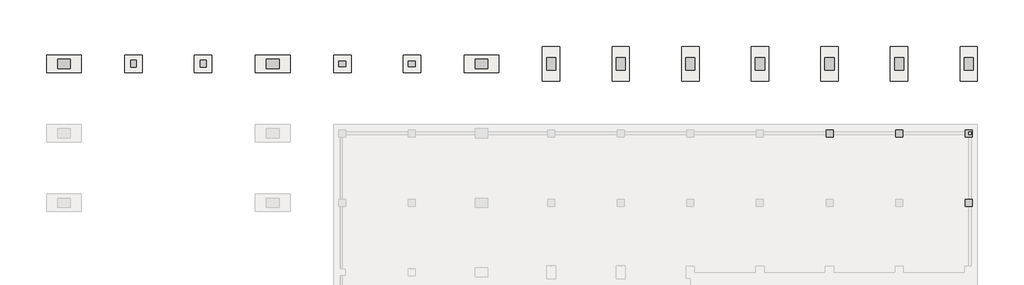
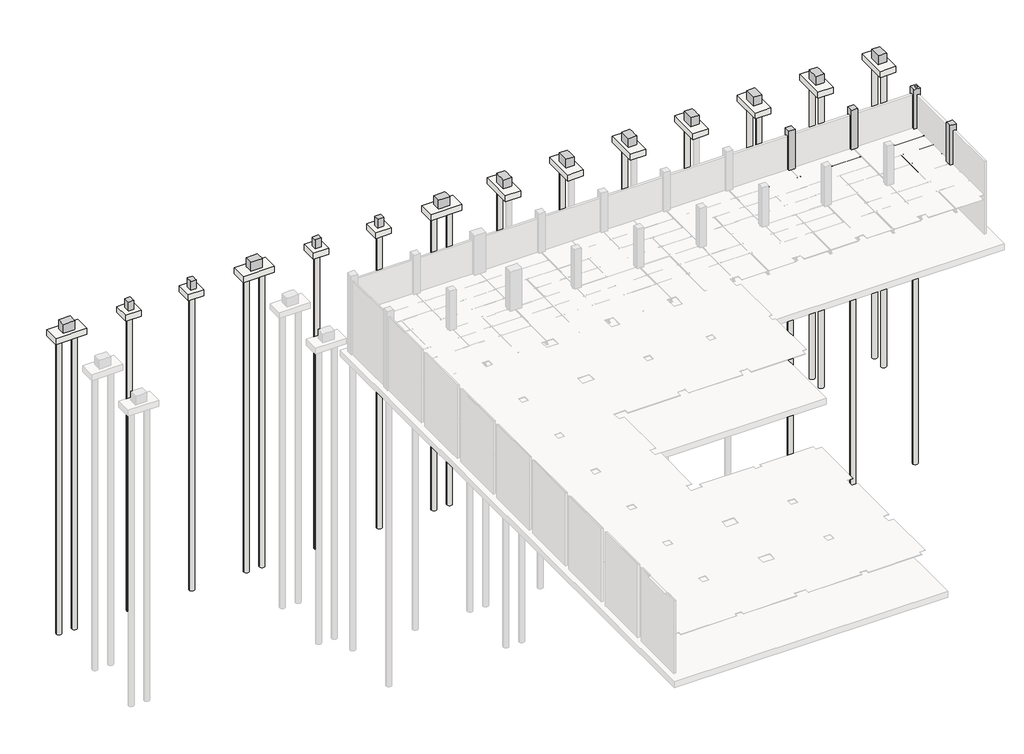
# Not in any storey, part 16 of 16: 37 slabs, 18 columns, 8 beams.
"""IFC4 building model written with IfcOpenShell, lengths in millimetres."""

from ifc_helpers import new_model, si_unit, point, frame, frame_2d, origin, place, context, project, spatial, polyline, circle_curve, trimmed, segment, composite_curve, outline, extrude, faceted_brep, element, save

model = new_model("IFC4")

# Units and contexts
model_context = context("Model", 3, world=origin())
ifc_project = project(units=[si_unit("LENGTHUNIT", "METRE", prefix="MILLI")], contexts=[model_context])

# Site, building
site = spatial("IfcSite", under=ifc_project)
building = spatial("IfcBuilding", under=site)

# Beams
placement = place(None, origin())
element("IfcBeam", 1, ObjectType="Steel Framing_C_KS : H_SB_AR_S02_C-150x75x6.5x10_J1", at=placement, inside=building, context=model_context, shape_type="SweptSolid", body=[
    extrude(outline(composite_curve([segment(polyline([(-7477.2, -3800.0381366), (-7477.2, -3950.0381366), (-7552.2, -3950.0381366)]), True, "CONTINUOUS"), segment(trimmed(circle_curve(frame_2d((-7542.2, -3950.0381366)), 10.0), [point((-7552.2, -3950.0381366))], [point((-7542.2, -3940.0381366))], False, "CARTESIAN"), True, "CONTINUOUS"), segment(polyline([(-7542.2, -3940.0381366), (-7483.7, -3930.7726469), (-7483.7, -3819.3036264), (-7542.2, -3810.0381366)]), True, "CONTINUOUS"), segment(trimmed(circle_curve(frame_2d((-7542.2, -3800.0381366)), 10.0), [point((-7542.2, -3810.0381366))], [point((-7552.2, -3800.0381366))], False, "CARTESIAN"), True, "CONTINUOUS"), segment(polyline([(-7552.2, -3800.0381366), (-7477.2, -3800.0381366)]), True, "CONTINUOUS")], self_intersect=False)), frame((63112.7, 0.0, 0.0), z_axis=(1.0, 0.0, 0.0), x_axis=(0.0, 1.0, 0.0)), (0.0, 0.0, 1.0), 2774.6),
])
element("IfcBeam", 2, ObjectType="Steel Framing_C_KS : H_SB_AR_S02_C-150x75x6.5x10_J1", at=placement, inside=building, context=model_context, shape_type="SweptSolid", body=[
    extrude(outline(composite_curve([segment(polyline([(-7477.2, -3800.0381366), (-7477.2, -3950.0381366), (-7552.2, -3950.0381366)]), True, "CONTINUOUS"), segment(trimmed(circle_curve(frame_2d((-7542.2, -3950.0381366)), 10.0), [point((-7552.2, -3950.0381366))], [point((-7542.2, -3940.0381366))], False, "CARTESIAN"), True, "CONTINUOUS"), segment(polyline([(-7542.2, -3940.0381366), (-7483.7, -3930.7726469), (-7483.7, -3819.3036264), (-7542.2, -3810.0381366)]), True, "CONTINUOUS"), segment(trimmed(circle_curve(frame_2d((-7542.2, -3800.0381366)), 10.0), [point((-7542.2, -3810.0381366))], [point((-7552.2, -3800.0381366))], False, "CARTESIAN"), True, "CONTINUOUS"), segment(polyline([(-7552.2, -3800.0381366), (-7477.2, -3800.0381366)]), True, "CONTINUOUS")], self_intersect=False)), frame((66112.7, 0.0, 0.0), z_axis=(1.0, 0.0, 0.0), x_axis=(0.0, 1.0, 0.0)), (0.0, 0.0, 1.0), 2774.6),
])
element("IfcBeam", 3, ObjectType="Steel Framing_C_KS : H_SB_AR_S02_C-150x75x6.5x10_J1", at=placement, inside=building, context=model_context, shape_type="SweptSolid", body=[
    extrude(outline(composite_curve([segment(polyline([(-7477.2, -3800.0381366), (-7477.2, -3950.0381366), (-7552.2, -3950.0381366)]), True, "CONTINUOUS"), segment(trimmed(circle_curve(frame_2d((-7542.2, -3950.0381366)), 10.0), [point((-7552.2, -3950.0381366))], [point((-7542.2, -3940.0381366))], False, "CARTESIAN"), True, "CONTINUOUS"), segment(polyline([(-7542.2, -3940.0381366), (-7483.7, -3930.7726469), (-7483.7, -3819.3036264), (-7542.2, -3810.0381366)]), True, "CONTINUOUS"), segment(trimmed(circle_curve(frame_2d((-7542.2, -3800.0381366)), 10.0), [point((-7542.2, -3810.0381366))], [point((-7552.2, -3800.0381366))], False, "CARTESIAN"), True, "CONTINUOUS"), segment(polyline([(-7552.2, -3800.0381366), (-7477.2, -3800.0381366)]), True, "CONTINUOUS")], self_intersect=False)), frame((69112.7, 0.0, 0.0), z_axis=(1.0, 0.0, 0.0), x_axis=(0.0, 1.0, 0.0)), (0.0, 0.0, 1.0), 2774.6),
])
element("IfcBeam", 4, ObjectType="Steel Framing_H_KS : H_SB_AR_S02_H-400x200x8x13_BSB1", at=placement, inside=building, context=model_context, shape_type="SweptSolid", body=[
    extrude(outline(composite_curve([segment(polyline([(-4187.0381366, 74900.0), (-4200.0381366, 74900.0), (-4200.0381366, 75100.0), (-4187.0381366, 75100.0), (-4187.0381366, 75020.0)]), True, "CONTINUOUS"), segment(trimmed(circle_curve(frame_2d((-4171.0381366, 75020.0)), 16.0), [point((-4187.0381366, 75020.0))], [point((-4171.0381366, 75004.0))], True, "CARTESIAN"), True, "CONTINUOUS"), segment(polyline([(-4171.0381366, 75004.0), (-3829.0381366, 75004.0)]), True, "CONTINUOUS"), segment(trimmed(circle_curve(frame_2d((-3829.0381366, 75020.0)), 16.0), [point((-3829.0381366, 75004.0))], [point((-3813.0381366, 75020.0))], True, "CARTESIAN"), True, "CONTINUOUS"), segment(polyline([(-3813.0381366, 75020.0), (-3813.0381366, 75100.0), (-3800.0381366, 75100.0), (-3800.0381366, 74900.0), (-3813.0381366, 74900.0), (-3813.0381366, 74980.0)]), True, "CONTINUOUS"), segment(trimmed(circle_curve(frame_2d((-3829.0381366, 74980.0)), 16.0), [point((-3813.0381366, 74980.0))], [point((-3829.0381366, 74996.0))], True, "CARTESIAN"), True, "CONTINUOUS"), segment(polyline([(-3829.0381366, 74996.0), (-4171.0381366, 74996.0)]), True, "CONTINUOUS"), segment(trimmed(circle_curve(frame_2d((-4171.0381366, 74980.0)), 16.0), [point((-4171.0381366, 74996.0))], [point((-4187.0381366, 74980.0))], True, "CARTESIAN"), True, "CONTINUOUS"), segment(polyline([(-4187.0381366, 74980.0), (-4187.0381366, 74900.0)]), True, "CONTINUOUS")], self_intersect=False)), frame((0.0, -11887.3, 0.0), z_axis=(0.0, 1.0, 0.0), x_axis=(0.0, 0.0, 1.0)), (0.0, 0.0, 1.0), 5887.3),
])
element("IfcBeam", 5, ObjectType="Steel Framing_C_KS : H_SB_AR_S02_C-150x75x6.5x10_J1", at=placement, inside=building, context=model_context, shape_type="SweptSolid", body=[
    extrude(outline(composite_curve([segment(polyline([(-7477.2, -3800.0381366), (-7477.2, -3950.0381366), (-7552.2, -3950.0381366)]), True, "CONTINUOUS"), segment(trimmed(circle_curve(frame_2d((-7542.2, -3950.0381366)), 10.0), [point((-7552.2, -3950.0381366))], [point((-7542.2, -3940.0381366))], False, "CARTESIAN"), True, "CONTINUOUS"), segment(polyline([(-7542.2, -3940.0381366), (-7483.7, -3930.7726469), (-7483.7, -3819.3036264), (-7542.2, -3810.0381366)]), True, "CONTINUOUS"), segment(trimmed(circle_curve(frame_2d((-7542.2, -3800.0381366)), 10.0), [point((-7542.2, -3810.0381366))], [point((-7552.2, -3800.0381366))], False, "CARTESIAN"), True, "CONTINUOUS"), segment(polyline([(-7552.2, -3800.0381366), (-7477.2, -3800.0381366)]), True, "CONTINUOUS")], self_intersect=False)), frame((72112.7, 0.0, 0.0), z_axis=(1.0, 0.0, 0.0), x_axis=(0.0, 1.0, 0.0)), (0.0, 0.0, 1.0), 2774.6),
])
element("IfcBeam", 6, ObjectType="Steel Framing_C_KS : H_SB_AR_S02_C-150x75x6.5x10_J1", at=placement, inside=building, context=model_context, shape_type="SweptSolid", body=[
    extrude(outline(composite_curve([segment(polyline([(-8977.2, -3800.0381366), (-8977.2, -3950.0381366), (-9052.2, -3950.0381366)]), True, "CONTINUOUS"), segment(trimmed(circle_curve(frame_2d((-9042.2, -3950.0381366)), 10.0), [point((-9052.2, -3950.0381366))], [point((-9042.2, -3940.0381366))], False, "CARTESIAN"), True, "CONTINUOUS"), segment(polyline([(-9042.2, -3940.0381366), (-8983.7, -3930.7726469), (-8983.7, -3819.3036264), (-9042.2, -3810.0381366)]), True, "CONTINUOUS"), segment(trimmed(circle_curve(frame_2d((-9042.2, -3800.0381366)), 10.0), [point((-9042.2, -3810.0381366))], [point((-9052.2, -3800.0381366))], False, "CARTESIAN"), True, "CONTINUOUS"), segment(polyline([(-9052.2, -3800.0381366), (-8977.2, -3800.0381366)]), True, "CONTINUOUS")], self_intersect=False)), frame((75112.7, 0.0, 0.0), z_axis=(1.0, 0.0, 0.0), x_axis=(0.0, 1.0, 0.0)), (0.0, 0.0, 1.0), 2887.3),
])
element("IfcBeam", 7, ObjectType="Steel Framing_C_KS : H_SB_AR_S02_C-150x75x6.5x10_J1", at=placement, inside=building, context=model_context, shape_type="SweptSolid", body=[
    extrude(outline(composite_curve([segment(polyline([(-10477.2, -3800.0381366), (-10477.2, -3950.0381366), (-10552.2, -3950.0381366)]), True, "CONTINUOUS"), segment(trimmed(circle_curve(frame_2d((-10542.2, -3950.0381366)), 10.0), [point((-10552.2, -3950.0381366))], [point((-10542.2, -3940.0381366))], False, "CARTESIAN"), True, "CONTINUOUS"), segment(polyline([(-10542.2, -3940.0381366), (-10483.7, -3930.7726469), (-10483.7, -3819.3036264), (-10542.2, -3810.0381366)]), True, "CONTINUOUS"), segment(trimmed(circle_curve(frame_2d((-10542.2, -3800.0381366)), 10.0), [point((-10542.2, -3810.0381366))], [point((-10552.2, -3800.0381366))], False, "CARTESIAN"), True, "CONTINUOUS"), segment(polyline([(-10552.2, -3800.0381366), (-10477.2, -3800.0381366)]), True, "CONTINUOUS")], self_intersect=False)), frame((75112.7, 0.0, 0.0), z_axis=(1.0, 0.0, 0.0), x_axis=(0.0, 1.0, 0.0)), (0.0, 0.0, 1.0), 2887.3),
])
element("IfcBeam", 8, ObjectType="Steel Framing_C_KS : H_SB_AR_S02_C-150x75x6.5x10_J1", at=placement, inside=building, context=model_context, shape_type="SweptSolid", body=[
    extrude(outline(composite_curve([segment(polyline([(-7477.2, -3800.0381366), (-7477.2, -3950.0381366), (-7552.2, -3950.0381366)]), True, "CONTINUOUS"), segment(trimmed(circle_curve(frame_2d((-7542.2, -3950.0381366)), 10.0), [point((-7552.2, -3950.0381366))], [point((-7542.2, -3940.0381366))], False, "CARTESIAN"), True, "CONTINUOUS"), segment(polyline([(-7542.2, -3940.0381366), (-7483.7, -3930.7726469), (-7483.7, -3819.3036264), (-7542.2, -3810.0381366)]), True, "CONTINUOUS"), segment(trimmed(circle_curve(frame_2d((-7542.2, -3800.0381366)), 10.0), [point((-7542.2, -3810.0381366))], [point((-7552.2, -3800.0381366))], False, "CARTESIAN"), True, "CONTINUOUS"), segment(polyline([(-7552.2, -3800.0381366), (-7477.2, -3800.0381366)]), True, "CONTINUOUS")], self_intersect=False)), frame((75112.7, 0.0, 0.0), z_axis=(1.0, 0.0, 0.0), x_axis=(0.0, 1.0, 0.0)), (0.0, 0.0, 1.0), 2887.3),
])

# Columns
element("IfcColumn", 9, ObjectType="RC_Column_Rectangular : H_SC_AR_S15_UG PED_Bit_800x1100_PD1", at=placement, inside=building, context=model_context, shape_type="Brep", body=[
    faceted_brep([(35450.0, 400.0, -700.0381366), (36550.0, 400.0, -700.0381366), (36550.0, -400.0, -700.0381366), (35450.0, -400.0, -700.0381366), (35450.0, 400.0, 199.9618634), (36550.0, 400.0, 199.9618634), (36550.0, 200.0, 199.9618634), (36550.0, -200.0, 199.9618634), (36550.0, -400.0, 199.9618634), (36550.0, -400.0, -0.0381366), (35450.0, -400.0, 199.9618634), (35450.0, -400.0, -0.0381366), (35450.0, -200.0, 199.9618634), (35450.0, 200.0, 199.9618634)], [[[0, 1, 2, 3]], [[4, 5, 1, 0]], [[5, 6, 7, 8, 9, 2, 1]], [[8, 10, 11, 3, 2, 9]], [[10, 12, 13, 4, 0, 3, 11]], [[4, 13, 12, 10, 8, 7, 6, 5]]]),
])
element("IfcColumn", 10, ObjectType="RC_Column_Rectangular : H_SC_AR_S15_UG PED_Bit_800x1100_PD1", at=placement, inside=building, context=model_context, shape_type="Brep", body=[
    faceted_brep([(42400.0, 550.0, -700.0381366), (42400.0, -550.0, -700.0381366), (41600.0, -550.0, -700.0381366), (41600.0, 550.0, -700.0381366), (42400.0, 550.0, 199.9618634), (42400.0, 200.0, 199.9618634), (42400.0, -200.0, 199.9618634), (42400.0, -550.0, 199.9618634), (42400.0, -550.0, -0.0381366), (41600.0, -550.0, 199.9618634), (41600.0, -550.0, -0.0381366), (41600.0, -200.0, 199.9618634), (41600.0, 200.0, 199.9618634), (41600.0, 550.0, 199.9618634)], [[[0, 1, 2, 3]], [[4, 5, 6, 7, 8, 1, 0]], [[7, 9, 10, 2, 1, 8]], [[9, 11, 12, 13, 3, 2, 10]], [[13, 4, 0, 3]], [[4, 13, 12, 11, 9, 7, 6, 5]]]),
])
element("IfcColumn", 11, ObjectType="RC_Column_Rectangular : H_SC_AR_S15_UG PED_Bit_800x1100_PD1", at=placement, inside=building, context=model_context, shape_type="Brep", body=[
    faceted_brep([(48400.0, 550.0, -700.0381366), (48400.0, -550.0, -700.0381366), (47600.0, -550.0, -700.0381366), (47600.0, 550.0, -700.0381366), (48400.0, 550.0, 199.9618634), (48400.0, 200.0, 199.9618634), (48400.0, -200.0, 199.9618634), (48400.0, -550.0, 199.9618634), (48400.0, -550.0, -0.0381366), (47600.0, -550.0, 199.9618634), (47600.0, -550.0, -0.0381366), (47600.0, -200.0, 199.9618634), (47600.0, 200.0, 199.9618634), (47600.0, 550.0, 199.9618634)], [[[0, 1, 2, 3]], [[4, 5, 6, 7, 8, 1, 0]], [[7, 9, 10, 2, 1, 8]], [[9, 11, 12, 13, 3, 2, 10]], [[13, 4, 0, 3]], [[4, 13, 12, 11, 9, 7, 6, 5]]]),
])
element("IfcColumn", 12, ObjectType="RC_Column_Rectangular : H_SC_AR_S15_UG PED_Bit_800x1100_PD1", at=placement, inside=building, context=model_context, shape_type="Brep", body=[
    faceted_brep([(54400.0, 550.0, -700.0381366), (54400.0, -550.0, -700.0381366), (53600.0, -550.0, -700.0381366), (53600.0, 550.0, -700.0381366), (54400.0, 550.0, 199.9618634), (54400.0, 200.0, 199.9618634), (54400.0, -200.0, 199.9618634), (54400.0, -550.0, 199.9618634), (54400.0, -550.0, -0.0381366), (53600.0, -550.0, 199.9618634), (53600.0, -550.0, -0.0381366), (53600.0, -200.0, 199.9618634), (53600.0, 200.0, 199.9618634), (53600.0, 550.0, 199.9618634)], [[[0, 1, 2, 3]], [[4, 5, 6, 7, 8, 1, 0]], [[7, 9, 10, 2, 1, 8]], [[9, 11, 12, 13, 3, 2, 10]], [[13, 4, 0, 3]], [[4, 13, 12, 11, 9, 7, 6, 5]]]),
])
element("IfcColumn", 13, ObjectType="RC_Column_Rectangular : H_SC_AR_S15_UG PED_Bit_800x1100_PD1", at=placement, inside=building, context=model_context, shape_type="Brep", body=[
    faceted_brep([(60400.0, 550.0, -700.0381366), (60400.0, -550.0, -700.0381366), (59600.0, -550.0, -700.0381366), (59600.0, 550.0, -700.0381366), (60400.0, 550.0, 199.9618634), (60400.0, 200.0, 199.9618634), (60400.0, -200.0, 199.9618634), (60400.0, -550.0, 199.9618634), (60400.0, -550.0, -0.0381366), (59600.0, -550.0, 199.9618634), (59600.0, -550.0, -0.0381366), (59600.0, -200.0, 199.9618634), (59600.0, 200.0, 199.9618634), (59600.0, 550.0, 199.9618634)], [[[0, 1, 2, 3]], [[4, 5, 6, 7, 8, 1, 0]], [[7, 9, 10, 2, 1, 8]], [[9, 11, 12, 13, 3, 2, 10]], [[13, 4, 0, 3]], [[4, 13, 12, 11, 9, 7, 6, 5]]]),
])
element("IfcColumn", 14, ObjectType="RC_Column_Rectangular : H_SC_AR_S15_UG PED_Bit_800x1100_PD1", at=placement, inside=building, context=model_context, shape_type="Brep", body=[
    faceted_brep([(66400.0, 550.0, -700.0381366), (66400.0, -550.0, -700.0381366), (65600.0, -550.0, -700.0381366), (65600.0, 550.0, -700.0381366), (66400.0, 550.0, 199.9618634), (66400.0, 200.0, 199.9618634), (66400.0, -200.0, 199.9618634), (66400.0, -550.0, 199.9618634), (66400.0, -550.0, -0.0381366), (65600.0, -550.0, 199.9618634), (65600.0, -550.0, -0.0381366), (65600.0, -200.0, 199.9618634), (65600.0, 200.0, 199.9618634), (65600.0, 550.0, 199.9618634)], [[[0, 1, 2, 3]], [[4, 5, 6, 7, 8, 1, 0]], [[7, 9, 10, 2, 1, 8]], [[9, 11, 12, 13, 3, 2, 10]], [[13, 4, 0, 3]], [[4, 13, 12, 11, 9, 7, 6, 5]]]),
])
element("IfcColumn", 15, ObjectType="RC_Column_Rectangular : H_SC_AR_S15_UG PED_Bit_800x1100_PD1", at=placement, inside=building, context=model_context, shape_type="Brep", body=[
    faceted_brep([(72400.0, 550.0, -700.0381366), (72400.0, -550.0, -700.0381366), (71600.0, -550.0, -700.0381366), (71600.0, 550.0, -700.0381366), (72400.0, 550.0, 199.9618634), (72400.0, 200.0, 199.9618634), (72400.0, -200.0, 199.9618634), (72400.0, -550.0, 199.9618634), (72400.0, -550.0, -0.0381366), (71600.0, -550.0, 199.9618634), (71600.0, -550.0, -0.0381366), (71600.0, -200.0, 199.9618634), (71600.0, 200.0, 199.9618634), (71600.0, 550.0, 199.9618634)], [[[0, 1, 2, 3]], [[4, 5, 6, 7, 8, 1, 0]], [[7, 9, 10, 2, 1, 8]], [[9, 11, 12, 13, 3, 2, 10]], [[13, 4, 0, 3]], [[4, 13, 12, 11, 9, 7, 6, 5]]]),
])
element("IfcColumn", 16, ObjectType="RC_Column_Rectangular : H_SC_AR_S15_UG PED_Bit_800x1100_PD1", at=placement, inside=building, context=model_context, shape_type="Brep", body=[
    faceted_brep([(78400.0, 550.0, -700.0381366), (78400.0, -550.0, -700.0381366), (77600.0, -550.0, -700.0381366), (77600.0, 550.0, -700.0381366), (78400.0, 550.0, 199.9618634), (78400.0, -550.0, 199.9618634), (78307.5526559, -550.0, 199.9618634), (78200.0, -550.0, 199.9618634), (77800.0, -550.0, 199.9618634), (77600.0, -550.0, 199.9618634), (77600.0, -550.0, -0.0381366), (77600.0, -200.0, 199.9618634), (77600.0, 550.0, 199.9618634)], [[[0, 1, 2, 3]], [[4, 5, 1, 0]], [[5, 6, 7, 8, 9, 10, 2, 1]], [[9, 11, 12, 3, 2, 10]], [[12, 4, 0, 3]], [[4, 12, 11, 9, 8, 7, 6, 5]]]),
])
element("IfcColumn", 17, ObjectType="RC_Column_Rectangular : H_SC_AR_S15_UG PED_Bit_800x1100_PD1", at=placement, inside=building, context=model_context, shape_type="Brep", body=[
    faceted_brep([(17450.0, 400.0, -700.0381366), (18550.0, 400.0, -700.0381366), (18550.0, -400.0, -700.0381366), (17450.0, -400.0, -700.0381366), (17450.0, 400.0, 199.9618634), (18550.0, 400.0, 199.9618634), (18550.0, 200.0, 199.9618634), (18550.0, -200.0, 199.9618634), (18550.0, -400.0, 199.9618634), (18550.0, -400.0, -0.0381366), (18200.0, -400.0, 199.9618634), (17800.0, -400.0, 199.9618634), (17450.0, -400.0, 199.9618634), (17450.0, -400.0, -0.0381366), (17450.0, -200.0, 199.9618634), (17450.0, 200.0, 199.9618634)], [[[0, 1, 2, 3]], [[4, 5, 1, 0]], [[5, 6, 7, 8, 9, 2, 1]], [[8, 10, 11, 12, 13, 3, 2, 9]], [[12, 14, 15, 4, 0, 3, 13]], [[4, 15, 14, 12, 11, 10, 8, 7, 6, 5]]]),
])
element("IfcColumn", 18, ObjectType="RC_Column_Rectangular : H_SC_AR_S15_UG PED_Bit_800x1100_PD1", at=placement, inside=building, context=model_context, shape_type="Brep", body=[
    faceted_brep([(-550.0, 400.0, -700.0381366), (550.0, 400.0, -700.0381366), (550.0, -400.0, -700.0381366), (-550.0, -400.0, -700.0381366), (-550.0, 400.0, 199.9618634), (550.0, 400.0, 199.9618634), (550.0, -200.0, 199.9618634), (550.0, -400.0, 199.9618634), (550.0, -400.0, -0.0381366), (200.0, -400.0, 199.9618634), (-550.0, -400.0, 199.9618634)], [[[0, 1, 2, 3]], [[4, 5, 1, 0]], [[5, 6, 7, 8, 2, 1]], [[7, 9, 10, 3, 2, 8]], [[10, 4, 0, 3]], [[4, 10, 9, 7, 6, 5]]]),
])
element("IfcColumn", 19, ObjectType="RC_Column_Rectangular : H_SC_AR_S15_UG PED_Bit_500x600_PD2", at=placement, inside=building, context=model_context, shape_type="Brep", body=[
    faceted_brep([(23700.0, 250.0, -700.0381366), (24300.0, 250.0, -700.0381366), (24300.0, -250.0, -700.0381366), (23700.0, -250.0, -700.0381366), (23700.0, 250.0, 199.9618634), (24300.0, 250.0, 199.9618634), (24300.0, 200.0, 199.9618634), (24300.0, -200.0, 199.9618634), (24300.0, -250.0, 199.9618634), (24300.0, -250.0, -0.0381366), (23700.0, -250.0, 199.9618634), (23700.0, -250.0, -0.0381366), (23700.0, -200.0, 199.9618634), (23700.0, 200.0, 199.9618634)], [[[0, 1, 2, 3]], [[4, 5, 1, 0]], [[5, 6, 7, 8, 9, 2, 1]], [[8, 10, 11, 3, 2, 9]], [[10, 12, 13, 4, 0, 3, 11]], [[4, 13, 12, 10, 8, 7, 6, 5]]]),
])
element("IfcColumn", 20, ObjectType="RC_Column_Rectangular : H_SC_AR_S15_UG PED_Bit_500x600_PD2", at=placement, inside=building, context=model_context, shape_type="Brep", body=[
    faceted_brep([(29700.0, 250.0, -700.0381366), (30300.0, 250.0, -700.0381366), (30300.0, -250.0, -700.0381366), (29700.0, -250.0, -700.0381366), (29700.0, 250.0, 199.9618634), (30300.0, 250.0, 199.9618634), (30300.0, 200.0, 199.9618634), (30300.0, -200.0, 199.9618634), (30300.0, -250.0, 199.9618634), (30300.0, -250.0, -0.0381366), (29700.0, -250.0, 199.9618634), (29700.0, -250.0, -0.0381366), (29700.0, -200.0, 199.9618634), (29700.0, 200.0, 199.9618634)], [[[0, 1, 2, 3]], [[4, 5, 1, 0]], [[5, 6, 7, 8, 9, 2, 1]], [[8, 10, 11, 3, 2, 9]], [[10, 12, 13, 4, 0, 3, 11]], [[4, 13, 12, 10, 8, 7, 6, 5]]]),
])
element("IfcColumn", 21, ObjectType="RC_Column_Rectangular : H_SC_AR_S15_UG PED_Bit_600x600_BC1", at=placement, inside=building, context=model_context, shape_type="Brep", body=[
    faceted_brep([(66300.0, -5700.0, -7800.0381366), (66300.0, -6300.0, -7800.0381366), (65700.0, -6300.0, -7800.0381366), (65700.0, -5700.0, -7800.0381366), (66300.0, -5700.0, 199.9618634), (66300.0, -6100.0, 199.9618634), (66300.0, -6300.0, 199.9618634), (66300.0, -6300.0, -0.0381366), (66300.0, -6300.0, -3800.0381366), (66300.0, -6300.0, -3832.0381366), (66300.0, -5700.0, -0.0381366), (66175.0, -6300.0, 199.9618634), (65825.0, -6300.0, 199.9618634), (65700.0, -6300.0, 199.9618634), (65700.0, -6300.0, -0.0381366), (65700.0, -6300.0, -3800.0381366), (65700.0, -6300.0, -3832.0381366), (65700.0, -6100.0, 199.9618634), (65700.0, -5700.0, 199.9618634), (65700.0, -5700.0, -0.0381366)], [[[0, 1, 2, 3]], [[4, 5, 6, 7, 8, 9, 1, 0, 10]], [[6, 11, 12, 13, 14, 15, 16, 2, 1, 9, 8, 7]], [[13, 17, 18, 19, 3, 2, 16, 15, 14]], [[18, 4, 10, 0, 3, 19]], [[4, 18, 17, 13, 12, 11, 6, 5]]]),
])
element("IfcColumn", 22, ObjectType="RC_Column_Rectangular : H_SC_AR_S15_UG PED_Bit_600x600_BC1", at=placement, inside=building, context=model_context, shape_type="Brep", body=[
    faceted_brep([(72300.0, -5700.0, -7800.0381366), (72300.0, -6300.0, -7800.0381366), (71700.0, -6300.0, -7800.0381366), (71700.0, -5700.0, -7800.0381366), (72300.0, -5700.0, 199.9618634), (72300.0, -6100.0, 199.9618634), (72300.0, -6300.0, 199.9618634), (72300.0, -6300.0, -0.0381366), (72300.0, -6300.0, -3800.0381366), (72300.0, -6300.0, -3832.0381366), (72300.0, -5700.0, -0.0381366), (72175.0, -6300.0, 199.9618634), (71825.0, -6300.0, 199.9618634), (71700.0, -6300.0, 199.9618634), (71700.0, -6300.0, -0.0381366), (71700.0, -6300.0, -3800.0381366), (71700.0, -6300.0, -3832.0381366), (71700.0, -6100.0, 199.9618634), (71700.0, -5700.0, 199.9618634), (71700.0, -5700.0, -0.0381366)], [[[0, 1, 2, 3]], [[4, 5, 6, 7, 8, 9, 1, 0, 10]], [[6, 11, 12, 13, 14, 15, 16, 2, 1, 9, 8, 7]], [[13, 17, 18, 19, 3, 2, 16, 15, 14]], [[18, 4, 10, 0, 3, 19]], [[4, 18, 17, 13, 12, 11, 6, 5]]]),
])
element("IfcColumn", 23, ObjectType="RC_Column_Rectangular : H_SC_AR_S15_UG PED_Bit_600x600_BC1", at=placement, inside=building, context=model_context, shape_type="Brep", body=[
    faceted_brep([(78300.0, -5700.0, -7800.0381366), (78300.0, -6300.0, -7800.0381366), (78200.0, -6300.0, -7800.0381366), (78000.0, -6300.0, -7800.0381366), (77700.0, -6300.0, -7800.0381366), (77700.0, -5700.0, -7800.0381366), (78300.0, -5700.0, 199.9618634), (78300.0, -6100.0, 199.9618634), (78300.0, -6300.0, 199.9618634), (78300.0, -5700.0, -0.0381366), (78200.0, -6300.0, 199.9618634), (78000.0, -6300.0, 199.9618634), (77800.0, -6300.0, 199.9618634), (77700.0, -6300.0, 199.9618634), (77700.0, -6300.0, -0.0381366), (77700.0, -6300.0, -3800.0381366), (77700.0, -6300.0, -3832.0381366), (77700.0, -6100.0, 199.9618634), (77700.0, -5700.0, 199.9618634), (77700.0, -5700.0, -0.0381366), (77800.0, -5700.0, 199.9618634), (78200.0, -5700.0, 199.9618634)], [[[0, 1, 2, 3, 4, 5]], [[6, 7, 8, 1, 0, 9]], [[8, 10, 11, 12, 13, 14, 15, 16, 4, 3, 2, 1]], [[13, 17, 18, 19, 5, 4, 16, 15, 14]], [[18, 20, 21, 6, 9, 0, 5, 19]], [[6, 21, 20, 18, 17, 13, 12, 11, 10, 8, 7]]]),
])
element("IfcColumn", 24, ObjectType="RC_Column_Rectangular : H_SC_AR_S15_UG PED_Bit_600x600_BC1", at=placement, inside=building, context=model_context, shape_type="Brep", body=[
    faceted_brep([(78300.0, -11700.0, -7800.0381366), (78300.0, -12300.0, -7800.0381366), (78200.0, -12300.0, -7800.0381366), (78000.0, -12300.0, -7800.0381366), (77700.0, -12300.0, -7800.0381366), (77700.0, -11700.0, -7800.0381366), (78000.0, -11700.0, -7800.0381366), (78200.0, -11700.0, -7800.0381366), (78300.0, -11700.0, 199.9618634), (78300.0, -12300.0, 199.9618634), (78200.0, -12300.0, 199.9618634), (78000.0, -12300.0, 199.9618634), (77800.0, -12300.0, 199.9618634), (77700.0, -12300.0, 199.9618634), (77700.0, -12300.0, -0.0381366), (77700.0, -12300.0, -3800.0381366), (77700.0, -12300.0, -3832.0381366), (77700.0, -12175.0, 199.9618634), (77700.0, -11825.0, 199.9618634), (77700.0, -11700.0, 199.9618634), (77700.0, -11700.0, -0.0381366), (77700.0, -11700.0, -3800.0381366), (77700.0, -11700.0, -3832.0381366), (77800.0, -11700.0, 199.9618634), (78000.0, -11700.0, 199.9618634), (78200.0, -11700.0, 199.9618634)], [[[0, 1, 2, 3, 4, 5, 6, 7]], [[8, 9, 1, 0]], [[9, 10, 11, 12, 13, 14, 15, 16, 4, 3, 2, 1]], [[13, 17, 18, 19, 20, 21, 22, 5, 4, 16, 15, 14]], [[19, 23, 24, 25, 8, 0, 7, 6, 5, 22, 21, 20]], [[8, 25, 24, 23, 19, 18, 17, 13, 12, 11, 10, 9]]]),
])
element("IfcColumn", 25, ObjectType="RC_Column_Rectangular : H_SC_AR_S15_UG PED_Bit_500x600_PD2", at=placement, inside=building, context=model_context, shape_type="Brep", body=[
    faceted_brep([(5750.0, -300.0, -700.0381366), (5750.0, 300.0, -700.0381366), (6250.0, 300.0, -700.0381366), (6250.0, -300.0, -700.0381366), (5750.0, -300.0, 199.9618634), (5750.0, -200.0, 199.9618634), (5750.0, 200.0, 199.9618634), (5750.0, 300.0, 199.9618634), (5750.0, -300.0, -0.0381366), (6250.0, 300.0, 199.9618634), (6250.0, 200.0, 199.9618634), (6250.0, -200.0, 199.9618634), (6250.0, -300.0, 199.9618634), (6250.0, -300.0, -0.0381366)], [[[0, 1, 2, 3]], [[4, 5, 6, 7, 1, 0, 8]], [[7, 9, 2, 1]], [[9, 10, 11, 12, 13, 3, 2]], [[12, 4, 8, 0, 3, 13]], [[4, 12, 11, 10, 9, 7, 6, 5]]]),
])
element("IfcColumn", 26, ObjectType="RC_Column_Rectangular : H_SC_AR_S15_UG PED_Bit_500x600_PD2", at=placement, inside=building, context=model_context, shape_type="Brep", body=[
    faceted_brep([(11750.0, -300.0, -700.0381366), (11750.0, 300.0, -700.0381366), (12250.0, 300.0, -700.0381366), (12250.0, -300.0, -700.0381366), (11750.0, -300.0, 199.9618634), (11750.0, -200.0, 199.9618634), (11750.0, 200.0, 199.9618634), (11750.0, 300.0, 199.9618634), (11750.0, -300.0, -0.0381366), (12250.0, 300.0, 199.9618634), (12250.0, 200.0, 199.9618634), (12250.0, -200.0, 199.9618634), (12250.0, -300.0, 199.9618634), (12250.0, -300.0, -0.0381366)], [[[0, 1, 2, 3]], [[4, 5, 6, 7, 1, 0, 8]], [[7, 9, 2, 1]], [[9, 10, 11, 12, 13, 3, 2]], [[12, 4, 8, 0, 3, 13]], [[4, 12, 11, 10, 9, 7, 6, 5]]]),
])

# Slabs
element("IfcSlab", 27, ObjectType="Foundation Rectangular (Non-Pile) : H_SF_AR_S18_Shallow Fdn_Bitumen_1500x3000xT600_F1", at=placement, inside=building, context=model_context, shape_type="SweptSolid", body=[
    extrude(outline(polyline([(1500.0, -750.0), (-1500.0, -750.0), (-1500.0, 750.0), (1500.0, 750.0), (1500.0, -750.0)])), frame((0.0, 0.0, -1300.0381366), z_axis=(0.0, 0.0, 1.0), x_axis=(1.0, 0.0, 0.0)), (0.0, 0.0, 1.0), 600.0),
])
element("IfcSlab", 28, ObjectType="Foundation Rectangular (Non-Pile) : H_SF_AR_S18_Shallow Fdn_Bitumen_1500x3000xT600_F1", at=placement, inside=building, context=model_context, shape_type="SweptSolid", body=[
    extrude(outline(polyline([(19500.0, -750.0), (16500.0, -750.0), (16500.0, 750.0), (19500.0, 750.0), (19500.0, -750.0)])), frame((0.0, 0.0, -1300.0381366), z_axis=(0.0, 0.0, 1.0), x_axis=(1.0, 0.0, 0.0)), (0.0, 0.0, 1.0), 600.0),
])
element("IfcSlab", 29, ObjectType="Foundation Rectangular (Non-Pile) : H_SF_AR_S18_Shallow Fdn_Bitumen_1500x3000xT600_F1", at=placement, inside=building, context=model_context, shape_type="SweptSolid", body=[
    extrude(outline(polyline([(37500.0, -750.0), (34500.0, -750.0), (34500.0, 750.0), (37500.0, 750.0), (37500.0, -750.0)])), frame((0.0, 0.0, -1300.0381366), z_axis=(0.0, 0.0, 1.0), x_axis=(1.0, 0.0, 0.0)), (0.0, 0.0, 1.0), 600.0),
])
element("IfcSlab", 30, ObjectType="Foundation Rectangular (Non-Pile) : H_SF_AR_S18_Shallow Fdn_Bitumen_1500x3000xT600_F1", at=placement, inside=building, context=model_context, shape_type="SweptSolid", body=[
    extrude(outline(polyline([(42750.0, 1500.0), (42750.0, -1500.0), (41250.0, -1500.0), (41250.0, 1500.0), (42750.0, 1500.0)])), frame((0.0, 0.0, -1300.0381366), z_axis=(0.0, 0.0, 1.0), x_axis=(1.0, 0.0, 0.0)), (0.0, 0.0, 1.0), 600.0),
])
element("IfcSlab", 31, ObjectType="Foundation Rectangular (Non-Pile) : H_SF_AR_S18_Shallow Fdn_Bitumen_1500x3000xT600_F1", at=placement, inside=building, context=model_context, shape_type="SweptSolid", body=[
    extrude(outline(polyline([(48750.0, 1500.0), (48750.0, -1500.0), (47250.0, -1500.0), (47250.0, 1500.0), (48750.0, 1500.0)])), frame((0.0, 0.0, -1300.0381366), z_axis=(0.0, 0.0, 1.0), x_axis=(1.0, 0.0, 0.0)), (0.0, 0.0, 1.0), 600.0),
])
element("IfcSlab", 32, ObjectType="Foundation Rectangular (Non-Pile) : H_SF_AR_S18_Shallow Fdn_Bitumen_1500x3000xT600_F1", at=placement, inside=building, context=model_context, shape_type="SweptSolid", body=[
    extrude(outline(polyline([(54750.0, 1500.0), (54750.0, -1500.0), (53250.0, -1500.0), (53250.0, 1500.0), (54750.0, 1500.0)])), frame((0.0, 0.0, -1300.0381366), z_axis=(0.0, 0.0, 1.0), x_axis=(1.0, 0.0, 0.0)), (0.0, 0.0, 1.0), 600.0),
])
element("IfcSlab", 33, ObjectType="Foundation Rectangular (Non-Pile) : H_SF_AR_S18_Shallow Fdn_Bitumen_1500x3000xT600_F1", at=placement, inside=building, context=model_context, shape_type="SweptSolid", body=[
    extrude(outline(polyline([(60750.0, 1500.0), (60750.0, -1500.0), (59250.0, -1500.0), (59250.0, 1500.0), (60750.0, 1500.0)])), frame((0.0, 0.0, -1300.0381366), z_axis=(0.0, 0.0, 1.0), x_axis=(1.0, 0.0, 0.0)), (0.0, 0.0, 1.0), 600.0),
])
element("IfcSlab", 34, ObjectType="Foundation Rectangular (Non-Pile) : H_SF_AR_S18_Shallow Fdn_Bitumen_1500x3000xT600_F1", at=placement, inside=building, context=model_context, shape_type="SweptSolid", body=[
    extrude(outline(polyline([(66750.0, 1500.0), (66750.0, -1500.0), (65250.0, -1500.0), (65250.0, 1500.0), (66750.0, 1500.0)])), frame((0.0, 0.0, -1300.0381366), z_axis=(0.0, 0.0, 1.0), x_axis=(1.0, 0.0, 0.0)), (0.0, 0.0, 1.0), 600.0),
])
element("IfcSlab", 35, ObjectType="Foundation Rectangular (Non-Pile) : H_SF_AR_S18_Shallow Fdn_Bitumen_1500x3000xT600_F1", at=placement, inside=building, context=model_context, shape_type="SweptSolid", body=[
    extrude(outline(polyline([(72750.0, 1500.0), (72750.0, -1500.0), (71250.0, -1500.0), (71250.0, 1500.0), (72750.0, 1500.0)])), frame((0.0, 0.0, -1300.0381366), z_axis=(0.0, 0.0, 1.0), x_axis=(1.0, 0.0, 0.0)), (0.0, 0.0, 1.0), 600.0),
])
element("IfcSlab", 36, ObjectType="Foundation Rectangular (Non-Pile) : H_SF_AR_S18_Shallow Fdn_Bitumen_1500x3000xT600_F1", at=placement, inside=building, context=model_context, shape_type="SweptSolid", body=[
    extrude(outline(polyline([(78750.0, 1500.0), (78750.0, -1500.0), (77250.0, -1500.0), (77250.0, 1500.0), (78750.0, 1500.0)])), frame((0.0, 0.0, -1300.0381366), z_axis=(0.0, 0.0, 1.0), x_axis=(1.0, 0.0, 0.0)), (0.0, 0.0, 1.0), 600.0),
])
element("IfcSlab", 37, ObjectType="Foundation Rectangular (Non-Pile) : H_SF_AR_S18_Shallow Fdn_Bitumen_1500x1500xT600_F2", at=placement, inside=building, context=model_context, shape_type="SweptSolid", body=[
    extrude(outline(polyline([(6750.0, -750.0), (5250.0, -750.0), (5250.0, 750.0), (6750.0, 750.0), (6750.0, -750.0)])), frame((0.0, 0.0, -1300.0381366), z_axis=(0.0, 0.0, 1.0), x_axis=(1.0, 0.0, 0.0)), (0.0, 0.0, 1.0), 600.0),
])
element("IfcSlab", 38, ObjectType="Foundation Rectangular (Non-Pile) : H_SF_AR_S18_Shallow Fdn_Bitumen_1500x1500xT600_F2", at=placement, inside=building, context=model_context, shape_type="SweptSolid", body=[
    extrude(outline(polyline([(12750.0, -750.0), (11250.0, -750.0), (11250.0, 750.0), (12750.0, 750.0), (12750.0, -750.0)])), frame((0.0, 0.0, -1300.0381366), z_axis=(0.0, 0.0, 1.0), x_axis=(1.0, 0.0, 0.0)), (0.0, 0.0, 1.0), 600.0),
])
element("IfcSlab", 39, ObjectType="Foundation Rectangular (Non-Pile) : H_SF_AR_S18_Shallow Fdn_Bitumen_1500x1500xT600_F2", at=placement, inside=building, context=model_context, shape_type="SweptSolid", body=[
    extrude(outline(polyline([(24750.0, -750.0), (23250.0, -750.0), (23250.0, 750.0), (24750.0, 750.0), (24750.0, -750.0)])), frame((0.0, 0.0, -1300.0381366), z_axis=(0.0, 0.0, 1.0), x_axis=(1.0, 0.0, 0.0)), (0.0, 0.0, 1.0), 600.0),
])
element("IfcSlab", 40, ObjectType="Foundation Rectangular (Non-Pile) : H_SF_AR_S18_Shallow Fdn_Bitumen_1500x1500xT600_F2", at=placement, inside=building, context=model_context, shape_type="SweptSolid", body=[
    extrude(outline(polyline([(30750.0, -750.0), (29250.0, -750.0), (29250.0, 750.0), (30750.0, 750.0), (30750.0, -750.0)])), frame((0.0, 0.0, -1300.0381366), z_axis=(0.0, 0.0, 1.0), x_axis=(1.0, 0.0, 0.0)), (0.0, 0.0, 1.0), 600.0),
])
element("IfcSlab", 41, ObjectType="PILE : H_SF_AR_S19_PHC Pile_Pre-boring_D500_L30", at=placement, inside=building, context=model_context, shape_type="SweptSolid", body=[
    extrude(outline(composite_curve([segment(trimmed(circle_curve(frame_2d((17250.0, 0.0)), 250.0), [point((17000.0, 0.0))], [point((17500.0, 0.0))], False, "CARTESIAN"), True, "CONTINUOUS"), segment(trimmed(circle_curve(frame_2d((17250.0, 0.0)), 250.0), [point((17500.0, 0.0))], [point((17000.0, 0.0))], False, "CARTESIAN"), True, "CONTINUOUS")], self_intersect=False)), frame((0.0, 0.0, -31300.0381366), z_axis=(0.0, 0.0, 1.0), x_axis=(1.0, 0.0, 0.0)), (0.0, 0.0, 1.0), 30000.0),
])
element("IfcSlab", 42, ObjectType="PILE : H_SF_AR_S19_PHC Pile_Pre-boring_D500_L30", at=placement, inside=building, context=model_context, shape_type="SweptSolid", body=[
    extrude(outline(composite_curve([segment(trimmed(circle_curve(frame_2d((18750.0, 0.0)), 250.0), [point((18500.0, 0.0))], [point((19000.0, 0.0))], False, "CARTESIAN"), True, "CONTINUOUS"), segment(trimmed(circle_curve(frame_2d((18750.0, 0.0)), 250.0), [point((19000.0, 0.0))], [point((18500.0, 0.0))], False, "CARTESIAN"), True, "CONTINUOUS")], self_intersect=False)), frame((0.0, 0.0, -31300.0381366), z_axis=(0.0, 0.0, 1.0), x_axis=(1.0, 0.0, 0.0)), (0.0, 0.0, 1.0), 30000.0),
])
element("IfcSlab", 43, ObjectType="PILE : H_SF_AR_S19_PHC Pile_Pre-boring_D500_L30", at=placement, inside=building, context=model_context, shape_type="SweptSolid", body=[
    extrude(outline(composite_curve([segment(trimmed(circle_curve(frame_2d((-750.0, 0.0)), 250.0), [point((-1000.0, 0.0))], [point((-500.0, 0.0))], False, "CARTESIAN"), True, "CONTINUOUS"), segment(trimmed(circle_curve(frame_2d((-750.0, 0.0)), 250.0), [point((-500.0, 0.0))], [point((-1000.0, 0.0))], False, "CARTESIAN"), True, "CONTINUOUS")], self_intersect=False)), frame((0.0, 0.0, -31300.0381366), z_axis=(0.0, 0.0, 1.0), x_axis=(1.0, 0.0, 0.0)), (0.0, 0.0, 1.0), 30000.0),
])
element("IfcSlab", 44, ObjectType="PILE : H_SF_AR_S19_PHC Pile_Pre-boring_D500_L30", at=placement, inside=building, context=model_context, shape_type="SweptSolid", body=[
    extrude(outline(composite_curve([segment(trimmed(circle_curve(frame_2d((750.0, 0.0)), 250.0), [point((500.0, 0.0))], [point((1000.0, 0.0))], False, "CARTESIAN"), True, "CONTINUOUS"), segment(trimmed(circle_curve(frame_2d((750.0, 0.0)), 250.0), [point((1000.0, 0.0))], [point((500.0, 0.0))], False, "CARTESIAN"), True, "CONTINUOUS")], self_intersect=False)), frame((0.0, 0.0, -31300.0381366), z_axis=(0.0, 0.0, 1.0), x_axis=(1.0, 0.0, 0.0)), (0.0, 0.0, 1.0), 30000.0),
])
element("IfcSlab", 45, ObjectType="PILE : H_SF_AR_S19_PHC Pile_Pre-boring_D500_L30", at=placement, inside=building, context=model_context, shape_type="SweptSolid", body=[
    extrude(outline(composite_curve([segment(trimmed(circle_curve(frame_2d((35250.0, 0.0)), 250.0), [point((35000.0, 0.0))], [point((35500.0, 0.0))], False, "CARTESIAN"), True, "CONTINUOUS"), segment(trimmed(circle_curve(frame_2d((35250.0, 0.0)), 250.0), [point((35500.0, 0.0))], [point((35000.0, 0.0))], False, "CARTESIAN"), True, "CONTINUOUS")], self_intersect=False)), frame((0.0, 0.0, -31300.0381366), z_axis=(0.0, 0.0, 1.0), x_axis=(1.0, 0.0, 0.0)), (0.0, 0.0, 1.0), 30000.0),
])
element("IfcSlab", 46, ObjectType="PILE : H_SF_AR_S19_PHC Pile_Pre-boring_D500_L30", at=placement, inside=building, context=model_context, shape_type="SweptSolid", body=[
    extrude(outline(composite_curve([segment(trimmed(circle_curve(frame_2d((36750.0, 0.0)), 250.0), [point((36500.0, 0.0))], [point((37000.0, 0.0))], False, "CARTESIAN"), True, "CONTINUOUS"), segment(trimmed(circle_curve(frame_2d((36750.0, 0.0)), 250.0), [point((37000.0, 0.0))], [point((36500.0, 0.0))], False, "CARTESIAN"), True, "CONTINUOUS")], self_intersect=False)), frame((0.0, 0.0, -31300.0381366), z_axis=(0.0, 0.0, 1.0), x_axis=(1.0, 0.0, 0.0)), (0.0, 0.0, 1.0), 30000.0),
])
element("IfcSlab", 47, ObjectType="PILE : H_SF_AR_S19_PHC Pile_Pre-boring_D500_L30", at=placement, inside=building, context=model_context, shape_type="SweptSolid", body=[
    extrude(outline(composite_curve([segment(trimmed(circle_curve(frame_2d((42000.0, 750.0)), 250.0), [point((41750.0, 750.0))], [point((42250.0, 750.0))], False, "CARTESIAN"), True, "CONTINUOUS"), segment(trimmed(circle_curve(frame_2d((42000.0, 750.0)), 250.0), [point((42250.0, 750.0))], [point((41750.0, 750.0))], False, "CARTESIAN"), True, "CONTINUOUS")], self_intersect=False)), frame((0.0, 0.0, -31300.0381366), z_axis=(0.0, 0.0, 1.0), x_axis=(1.0, 0.0, 0.0)), (0.0, 0.0, 1.0), 30000.0),
])
element("IfcSlab", 48, ObjectType="PILE : H_SF_AR_S19_PHC Pile_Pre-boring_D500_L30", at=placement, inside=building, context=model_context, shape_type="SweptSolid", body=[
    extrude(outline(composite_curve([segment(trimmed(circle_curve(frame_2d((48000.0, 750.0)), 250.0), [point((47750.0, 750.0))], [point((48250.0, 750.0))], False, "CARTESIAN"), True, "CONTINUOUS"), segment(trimmed(circle_curve(frame_2d((48000.0, 750.0)), 250.0), [point((48250.0, 750.0))], [point((47750.0, 750.0))], False, "CARTESIAN"), True, "CONTINUOUS")], self_intersect=False)), frame((0.0, 0.0, -31300.0381366), z_axis=(0.0, 0.0, 1.0), x_axis=(1.0, 0.0, 0.0)), (0.0, 0.0, 1.0), 30000.0),
])
element("IfcSlab", 49, ObjectType="PILE : H_SF_AR_S19_PHC Pile_Pre-boring_D500_L30", at=placement, inside=building, context=model_context, shape_type="SweptSolid", body=[
    extrude(outline(composite_curve([segment(trimmed(circle_curve(frame_2d((54000.0, 750.0)), 250.0), [point((53750.0, 750.0))], [point((54250.0, 750.0))], False, "CARTESIAN"), True, "CONTINUOUS"), segment(trimmed(circle_curve(frame_2d((54000.0, 750.0)), 250.0), [point((54250.0, 750.0))], [point((53750.0, 750.0))], False, "CARTESIAN"), True, "CONTINUOUS")], self_intersect=False)), frame((0.0, 0.0, -31300.0381366), z_axis=(0.0, 0.0, 1.0), x_axis=(1.0, 0.0, 0.0)), (0.0, 0.0, 1.0), 30000.0),
])
element("IfcSlab", 50, ObjectType="PILE : H_SF_AR_S19_PHC Pile_Pre-boring_D500_L30", at=placement, inside=building, context=model_context, shape_type="SweptSolid", body=[
    extrude(outline(composite_curve([segment(trimmed(circle_curve(frame_2d((60000.0, 750.0)), 250.0), [point((59750.0, 750.0))], [point((60250.0, 750.0))], False, "CARTESIAN"), True, "CONTINUOUS"), segment(trimmed(circle_curve(frame_2d((60000.0, 750.0)), 250.0), [point((60250.0, 750.0))], [point((59750.0, 750.0))], False, "CARTESIAN"), True, "CONTINUOUS")], self_intersect=False)), frame((0.0, 0.0, -31300.0381366), z_axis=(0.0, 0.0, 1.0), x_axis=(1.0, 0.0, 0.0)), (0.0, 0.0, 1.0), 30000.0),
])
element("IfcSlab", 51, ObjectType="PILE : H_SF_AR_S19_PHC Pile_Pre-boring_D500_L30", at=placement, inside=building, context=model_context, shape_type="SweptSolid", body=[
    extrude(outline(composite_curve([segment(trimmed(circle_curve(frame_2d((66000.0, 750.0)), 250.0), [point((65750.0, 750.0))], [point((66250.0, 750.0))], False, "CARTESIAN"), True, "CONTINUOUS"), segment(trimmed(circle_curve(frame_2d((66000.0, 750.0)), 250.0), [point((66250.0, 750.0))], [point((65750.0, 750.0))], False, "CARTESIAN"), True, "CONTINUOUS")], self_intersect=False)), frame((0.0, 0.0, -31300.0381366), z_axis=(0.0, 0.0, 1.0), x_axis=(1.0, 0.0, 0.0)), (0.0, 0.0, 1.0), 30000.0),
])
element("IfcSlab", 52, ObjectType="PILE : H_SF_AR_S19_PHC Pile_Pre-boring_D500_L30", at=placement, inside=building, context=model_context, shape_type="SweptSolid", body=[
    extrude(outline(composite_curve([segment(trimmed(circle_curve(frame_2d((66000.0, -750.0)), 250.0), [point((65750.0, -750.0))], [point((66250.0, -750.0))], False, "CARTESIAN"), True, "CONTINUOUS"), segment(trimmed(circle_curve(frame_2d((66000.0, -750.0)), 250.0), [point((66250.0, -750.0))], [point((65750.0, -750.0))], False, "CARTESIAN"), True, "CONTINUOUS")], self_intersect=False)), frame((0.0, 0.0, -31300.0381366), z_axis=(0.0, 0.0, 1.0), x_axis=(1.0, 0.0, 0.0)), (0.0, 0.0, 1.0), 30000.0),
])
element("IfcSlab", 53, ObjectType="PILE : H_SF_AR_S19_PHC Pile_Pre-boring_D500_L30", at=placement, inside=building, context=model_context, shape_type="SweptSolid", body=[
    extrude(outline(composite_curve([segment(trimmed(circle_curve(frame_2d((72000.0, 750.0)), 250.0), [point((71750.0, 750.0))], [point((72250.0, 750.0))], False, "CARTESIAN"), True, "CONTINUOUS"), segment(trimmed(circle_curve(frame_2d((72000.0, 750.0)), 250.0), [point((72250.0, 750.0))], [point((71750.0, 750.0))], False, "CARTESIAN"), True, "CONTINUOUS")], self_intersect=False)), frame((0.0, 0.0, -31300.0381366), z_axis=(0.0, 0.0, 1.0), x_axis=(1.0, 0.0, 0.0)), (0.0, 0.0, 1.0), 30000.0),
])
element("IfcSlab", 54, ObjectType="PILE : H_SF_AR_S19_PHC Pile_Pre-boring_D500_L30", at=placement, inside=building, context=model_context, shape_type="SweptSolid", body=[
    extrude(outline(composite_curve([segment(trimmed(circle_curve(frame_2d((72000.0, -750.0)), 250.0), [point((71750.0, -750.0))], [point((72250.0, -750.0))], False, "CARTESIAN"), True, "CONTINUOUS"), segment(trimmed(circle_curve(frame_2d((72000.0, -750.0)), 250.0), [point((72250.0, -750.0))], [point((71750.0, -750.0))], False, "CARTESIAN"), True, "CONTINUOUS")], self_intersect=False)), frame((0.0, 0.0, -31300.0381366), z_axis=(0.0, 0.0, 1.0), x_axis=(1.0, 0.0, 0.0)), (0.0, 0.0, 1.0), 30000.0),
])
element("IfcSlab", 55, ObjectType="PILE : H_SF_AR_S19_PHC Pile_Pre-boring_D500_L30", at=placement, inside=building, context=model_context, shape_type="SweptSolid", body=[
    extrude(outline(composite_curve([segment(trimmed(circle_curve(frame_2d((78000.0, 750.0)), 250.0), [point((77750.0, 750.0))], [point((78250.0, 750.0))], False, "CARTESIAN"), True, "CONTINUOUS"), segment(trimmed(circle_curve(frame_2d((78000.0, 750.0)), 250.0), [point((78250.0, 750.0))], [point((77750.0, 750.0))], False, "CARTESIAN"), True, "CONTINUOUS")], self_intersect=False)), frame((0.0, 0.0, -31300.0381366), z_axis=(0.0, 0.0, 1.0), x_axis=(1.0, 0.0, 0.0)), (0.0, 0.0, 1.0), 30000.0),
])
element("IfcSlab", 56, ObjectType="PILE : H_SF_AR_S19_PHC Pile_Pre-boring_D500_L30", at=placement, inside=building, context=model_context, shape_type="SweptSolid", body=[
    extrude(outline(composite_curve([segment(trimmed(circle_curve(frame_2d((78000.0, -750.0)), 250.0), [point((77750.0, -750.0))], [point((78250.0, -750.0))], False, "CARTESIAN"), True, "CONTINUOUS"), segment(trimmed(circle_curve(frame_2d((78000.0, -750.0)), 250.0), [point((78250.0, -750.0))], [point((77750.0, -750.0))], False, "CARTESIAN"), True, "CONTINUOUS")], self_intersect=False)), frame((0.0, 0.0, -31300.0381366), z_axis=(0.0, 0.0, 1.0), x_axis=(1.0, 0.0, 0.0)), (0.0, 0.0, 1.0), 30000.0),
])
element("IfcSlab", 57, ObjectType="PILE : H_SF_AR_S19_PHC Pile_Pre-boring_D500_L30", at=placement, inside=building, context=model_context, shape_type="SweptSolid", body=[
    extrude(outline(composite_curve([segment(trimmed(circle_curve(frame_2d((30000.0, 0.0)), 250.0), [point((29750.0, 0.0))], [point((30250.0, 0.0))], False, "CARTESIAN"), True, "CONTINUOUS"), segment(trimmed(circle_curve(frame_2d((30000.0, 0.0)), 250.0), [point((30250.0, 0.0))], [point((29750.0, 0.0))], False, "CARTESIAN"), True, "CONTINUOUS")], self_intersect=False)), frame((0.0, 0.0, -31300.0381366), z_axis=(0.0, 0.0, 1.0), x_axis=(1.0, 0.0, 0.0)), (0.0, 0.0, 1.0), 30000.0),
])
element("IfcSlab", 58, ObjectType="PILE : H_SF_AR_S19_PHC Pile_Pre-boring_D500_L30", at=placement, inside=building, context=model_context, shape_type="SweptSolid", body=[
    extrude(outline(composite_curve([segment(trimmed(circle_curve(frame_2d((24000.0, 0.0)), 250.0), [point((23750.0, 0.0))], [point((24250.0, 0.0))], False, "CARTESIAN"), True, "CONTINUOUS"), segment(trimmed(circle_curve(frame_2d((24000.0, 0.0)), 250.0), [point((24250.0, 0.0))], [point((23750.0, 0.0))], False, "CARTESIAN"), True, "CONTINUOUS")], self_intersect=False)), frame((0.0, 0.0, -31300.0381366), z_axis=(0.0, 0.0, 1.0), x_axis=(1.0, 0.0, 0.0)), (0.0, 0.0, 1.0), 30000.0),
])
element("IfcSlab", 59, ObjectType="PILE : H_SF_AR_S19_PHC Pile_Pre-boring_D500_L30", at=placement, inside=building, context=model_context, shape_type="SweptSolid", body=[
    extrude(outline(composite_curve([segment(trimmed(circle_curve(frame_2d((12000.0, 0.0)), 250.0), [point((11750.0, 0.0))], [point((12250.0, 0.0))], False, "CARTESIAN"), True, "CONTINUOUS"), segment(trimmed(circle_curve(frame_2d((12000.0, 0.0)), 250.0), [point((12250.0, 0.0))], [point((11750.0, 0.0))], False, "CARTESIAN"), True, "CONTINUOUS")], self_intersect=False)), frame((0.0, 0.0, -31300.0381366), z_axis=(0.0, 0.0, 1.0), x_axis=(1.0, 0.0, 0.0)), (0.0, 0.0, 1.0), 30000.0),
])
element("IfcSlab", 60, ObjectType="PILE : H_SF_AR_S19_PHC Pile_Pre-boring_D500_L30", at=placement, inside=building, context=model_context, shape_type="SweptSolid", body=[
    extrude(outline(composite_curve([segment(trimmed(circle_curve(frame_2d((6000.0, 0.0)), 250.0), [point((5750.0, 0.0))], [point((6250.0, 0.0))], False, "CARTESIAN"), True, "CONTINUOUS"), segment(trimmed(circle_curve(frame_2d((6000.0, 0.0)), 250.0), [point((6250.0, 0.0))], [point((5750.0, 0.0))], False, "CARTESIAN"), True, "CONTINUOUS")], self_intersect=False)), frame((0.0, 0.0, -31300.0381366), z_axis=(0.0, 0.0, 1.0), x_axis=(1.0, 0.0, 0.0)), (0.0, 0.0, 1.0), 30000.0),
])
element("IfcSlab", 61, ObjectType="PILE : H_SF_AR_S19_PHC Pile_Pre-boring_D500_L30", at=placement, inside=building, context=model_context, shape_type="SweptSolid", body=[
    extrude(outline(composite_curve([segment(trimmed(circle_curve(frame_2d((66000.0, -6000.0)), 250.0), [point((65750.0, -6000.0))], [point((66250.0, -6000.0))], False, "CARTESIAN"), True, "CONTINUOUS"), segment(trimmed(circle_curve(frame_2d((66000.0, -6000.0)), 250.0), [point((66250.0, -6000.0))], [point((65750.0, -6000.0))], False, "CARTESIAN"), True, "CONTINUOUS")], self_intersect=False)), frame((0.0, 0.0, -37950.0381366), z_axis=(0.0, 0.0, 1.0), x_axis=(1.0, 0.0, 0.0)), (0.0, 0.0, 1.0), 29550.0),
])
element("IfcSlab", 62, ObjectType="PILE : H_SF_AR_S19_PHC Pile_Pre-boring_D500_L30", at=placement, inside=building, context=model_context, shape_type="SweptSolid", body=[
    extrude(outline(composite_curve([segment(trimmed(circle_curve(frame_2d((72000.0, -6000.0)), 250.0), [point((71750.0, -6000.0))], [point((72250.0, -6000.0))], False, "CARTESIAN"), True, "CONTINUOUS"), segment(trimmed(circle_curve(frame_2d((72000.0, -6000.0)), 250.0), [point((72250.0, -6000.0))], [point((71750.0, -6000.0))], False, "CARTESIAN"), True, "CONTINUOUS")], self_intersect=False)), frame((0.0, 0.0, -37950.0381366), z_axis=(0.0, 0.0, 1.0), x_axis=(1.0, 0.0, 0.0)), (0.0, 0.0, 1.0), 29550.0),
])
element("IfcSlab", 63, ObjectType="PILE : H_SF_AR_S19_PHC Pile_Pre-boring_D500_L30", at=placement, inside=building, context=model_context, shape_type="SweptSolid", body=[
    extrude(outline(composite_curve([segment(trimmed(circle_curve(frame_2d((78000.0, -6000.0)), 250.0), [point((77750.0, -6000.0))], [point((78250.0, -6000.0))], False, "CARTESIAN"), True, "CONTINUOUS"), segment(trimmed(circle_curve(frame_2d((78000.0, -6000.0)), 250.0), [point((78250.0, -6000.0))], [point((77750.0, -6000.0))], False, "CARTESIAN"), True, "CONTINUOUS")], self_intersect=False)), frame((0.0, 0.0, -37950.0381366), z_axis=(0.0, 0.0, 1.0), x_axis=(1.0, 0.0, 0.0)), (0.0, 0.0, 1.0), 29550.0),
])

save(model, "model.ifc")

# Revit data of these elements
# Type "Steel Framing_C_KS : H_SB_AR_S02_C-150x75x6.5x10_J1"
#   Type Mark = "J1"
#   H_SectionID = "C-150x75x6.5x10"
#   Assembly Code = "B10"
#   H_Ratio for Additional Steel Plate = 0.2
#   Perimeter = 0.51 m²/m
#   Nominal Weight = 18.60 kgf/m
#   Length [instance default] = 1000 mm
#   bf = 75 mm
#   d = 150 mm
#   tf = 10 mm
#   tw = 6.5 mm
#   x = 22.8 mm
#   A = 0.002371 m²
#   Structural Material [instance default] = Steel, 45-345
# Type "Steel Framing_H_KS : H_SB_AR_S02_H-400x200x8x13_BSB1"
#   Type Comments = "MAIN"
#   Type Mark = "BSB1"
#   H_SectionID = "H-400x200x8x13"
#   H_Ratio for Additional Steel Plate = 0.2
#   Width = 20.0 cm
#   Web Thickness = 0.8 cm
#   Web Fillet = 1.6 cm
#   Warping Constant = 649000.0 cm⁶
#   Torsional Moment of Inertia = 35.8981 cm⁴
#   Section Area = 84.12 cm²
#   Plastic Modulus weak axis = 268.0 cm³
#   Plastic Modulus strong axis = 1330.0 cm³
#   Perimeter = 1.56 m²/m
#   Nominal Weight = 66.00 kgf/m
#   Moment of Inertia weak axis = 1740.00 cm⁴
#   Moment of Inertia strong axis = 23700.00 cm⁴
#   Height = 40.0 cm
#   Flange Thickness = 1.3 cm
#   Elastic Modulus weak axis = 174.0 cm³
#   Elastic Modulus strong axis = 1190.0 cm³
#   Centroid Vertical = 20.0 cm
#   Centroid Horizontal = 10.0 cm
#   Bolt Spacing = 8.89 cm
#   Length [instance default] = 1500 mm
#   Structural Material [instance default] = Steel, 45-345
#   Section Name Key = ""
#   Assembly Code = ""
# Type "RC_Column_Rectangular : H_SC_AR_S15_UG PED_Bit_800x1100_PD1"
#   Type Mark = "PD1"
#   Type Comments = "UG"
#   H_SectionID = "600 x 900"
#   H_Rebar Ratio = 0.3
#   Width = 800 mm
#   Depth = 1100 mm
#   hec_material3 [instance default] = none
#   hec_material2 [instance default] = none
#   hec_material1 [instance default] = none
#   Structural Material [instance default] = none
#   Description = (empty or 0)
# Type "RC_Column_Rectangular : H_SC_AR_S15_UG PED_Bit_500x600_PD2"
#   Type Mark = "PD2"
#   Type Comments = "UG"
#   H_SectionID = "600 x 900"
#   H_Rebar Ratio = 0.3
#   Width = 500 mm
#   Depth = 600 mm
#   hec_material3 [instance default] = none
#   hec_material2 [instance default] = none
#   hec_material1 [instance default] = none
#   Structural Material [instance default] = none
#   Description = (empty or 0)
# Type "RC_Column_Rectangular : H_SC_AR_S15_UG PED_Bit_600x600_BC1"
#   Type Mark = "BC1"
#   Type Comments = "UG"
#   H_SectionID = "600 x 600"
#   H_Rebar Ratio = 0.3
#   Width = 600 mm
#   Depth = 600 mm
#   hec_material3 [instance default] = none
#   hec_material2 [instance default] = none
#   hec_material1 [instance default] = none
#   Structural Material [instance default] = none
#   Description = (empty or 0)
# Type "Foundation Rectangular (Non-Pile) : H_SF_AR_S18_Shallow Fdn_Bitumen_1500x3000xT600_F1"
#   Type Comments = "UG"
#   Type Mark = "F1"
#   Top bar = "D25@300"
#   Description = "UG Shallow Foundation"
#   Bottom bar = "D20@300"
#   H_Rebar Ratio = 0.12
#   Width = 1500 mm
#   Length = 3000 mm
#   Foundation Thickness = 600 mm
#   Structural Material [instance default] = none
#   Assembly Code = ""
# Type "Foundation Rectangular (Non-Pile) : H_SF_AR_S18_Shallow Fdn_Bitumen_1500x1500xT600_F2"
#   Type Comments = "UG"
#   Type Mark = "F2"
#   Top bar = "D25@300"
#   Description = "UG Shallow Foundation"
#   Bottom bar = "D20@300"
#   H_Rebar Ratio = 0.12
#   Width = 1500 mm
#   Length = 1500 mm
#   Foundation Thickness = 600 mm
#   Structural Material [instance default] = none
#   Assembly Code = ""
# Type "PILE : H_SF_AR_S19_PHC Pile_Pre-boring_D500_L30"
#   Assembly Code = "A1020120"
#   반지름 = 250 mm
#   최소 내포 = 150 mm
#   Diameter = 500 mm
#   Depth = 30000 mm
#   Structural Material [instance default] = none
# Elements 1, 2, 3, 5, 6, 7, 8 (IfcBeam, "Steel Framing_C_KS : H_SB_AR_S02_C-150x75x6.5x10_J1")
#   Structural Material = Steel, 45-345
#   Phase Created = New Construction
#   Materials on its faces: "Steel, 45-345"
# Element 4 (IfcBeam, "Steel Framing_H_KS : H_SB_AR_S02_H-400x200x8x13_BSB1")
#   Structural Material = Steel, 45-345
#   Phase Created = New Construction
#   Materials on its faces: "Steel, 45-345"
# Elements 9, 10, 11, 12, 13, 14, 15, 16, 17, 18 (IfcColumn, "RC_Column_Rectangular : H_SC_AR_S15_UG PED_Bit_800x1100_PD1")
#   Comments = ""
#   hec_material3 = none
#   hec_material2 = none
#   hec_material1 = none
#   Structural Material = 00_Concrete_Reinf. Conc.
#   Phase Created = New Construction
#   Materials on its faces: "00_Concrete_Reinf. Conc."
# Elements 19, 20, 25, 26 (IfcColumn, "RC_Column_Rectangular : H_SC_AR_S15_UG PED_Bit_500x600_PD2")
#   Comments = ""
#   hec_material3 = none
#   hec_material2 = none
#   hec_material1 = none
#   Structural Material = 00_Concrete_Reinf. Conc.
#   Phase Created = New Construction
#   Materials on its faces: "00_Concrete_Reinf. Conc."
# Elements 21, 22, 23, 24 (IfcColumn, "RC_Column_Rectangular : H_SC_AR_S15_UG PED_Bit_600x600_BC1")
#   Comments = ""
#   hec_material3 = none
#   hec_material2 = none
#   hec_material1 = none
#   Structural Material = 00_Concrete_Reinf. Conc.
#   Phase Created = New Construction
#   Materials on its faces: "00_Concrete_Reinf. Conc."
# Elements 27, 28, 29 (IfcSlab, "Foundation Rectangular (Non-Pile) : H_SF_AR_S18_Shallow Fdn_Bitumen_1500x3000xT600_F1")
#   Comments = ""
#   Structural Material = 00_Concrete_Reinf. Conc.
#   Phase Created = New Construction
#   Materials on its faces: "00_Concrete_Reinf. Conc."
# Elements 30, 31, 32, 33, 34, 35, 36 (IfcSlab, "Foundation Rectangular (Non-Pile) : H_SF_AR_S18_Shallow Fdn_Bitumen_1500x3000xT600_F1")
#   Structural Material = 00_Concrete_Reinf. Conc.
#   Phase Created = New Construction
#   Materials on its faces: "00_Concrete_Reinf. Conc."
# Elements 37, 38, 39, 40 (IfcSlab, "Foundation Rectangular (Non-Pile) : H_SF_AR_S18_Shallow Fdn_Bitumen_1500x1500xT600_F2")
#   Comments = ""
#   Structural Material = 00_Concrete_Reinf. Conc.
#   Phase Created = New Construction
#   Materials on its faces: "00_Concrete_Reinf. Conc."
